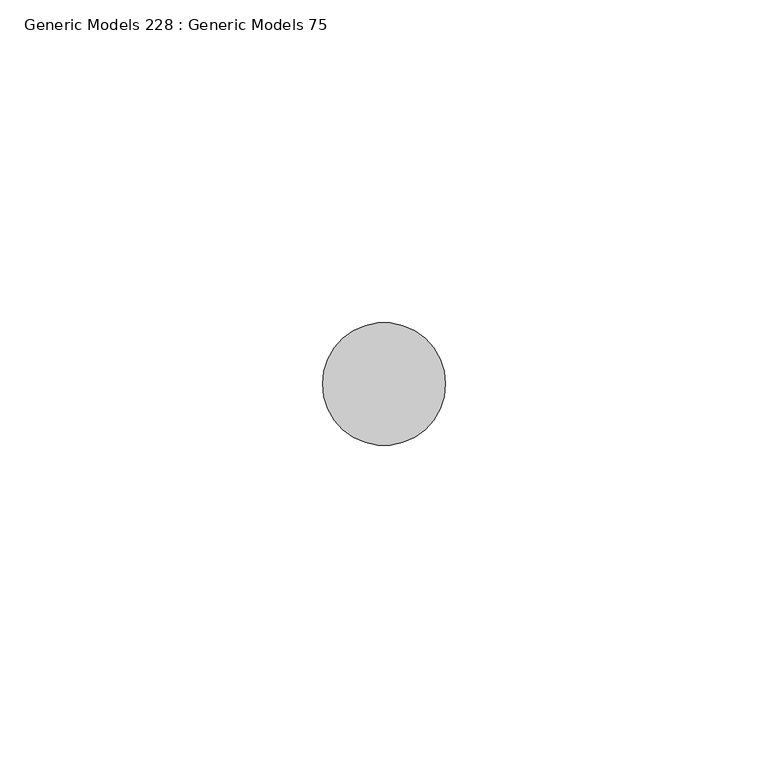
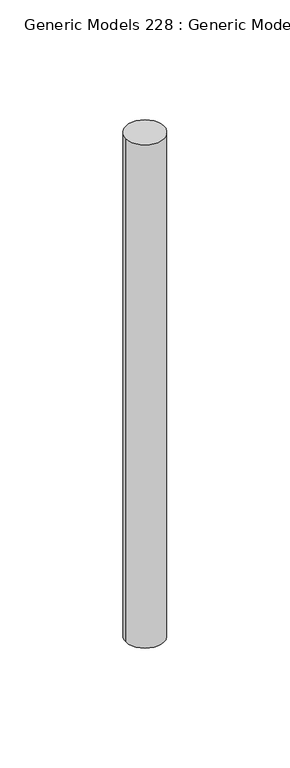
"""IFC4 building model written with IfcOpenShell, lengths in millimetres: proxy geometry, Generic Models 228 : Generic Models 75."""

from ifc_helpers import new_model, si_unit, point, frame, frame_2d, origin, place, context, project, spatial, circle_curve, trimmed, segment, composite_curve, outline, extrude, source, transform, mapped, element, save


def generic_models_228_generic_models_75_c9aeced4(model_context):
    return source(origin(), model_context, "Body", "SweptSolid", [
        extrude(outline(composite_curve([segment(trimmed(circle_curve(frame_2d((31988.1215778, 35167.5357185)), 9.525), [point((31978.5965778, 35167.5357185))], [point((31997.6465778, 35167.5357185))], False, "CARTESIAN"), True, "CONTINUOUS"), segment(trimmed(circle_curve(frame_2d((31988.1215778, 35167.5357185)), 9.525), [point((31997.6465778, 35167.5357185))], [point((31978.5965778, 35167.5357185))], False, "CARTESIAN"), True, "CONTINUOUS")], self_intersect=False)), frame((0.0, 0.0, 266172.95), z_axis=(0.0, 0.0, 1.0), x_axis=(1.0, 0.0, 0.0)), (0.0, 0.0, 1.0), 266.7),
    ])


if __name__ == "__main__":
    model = new_model("IFC4")
    model_context = context("Model", 3, world=origin())
    ifc_project = project(units=[si_unit("LENGTHUNIT", "METRE", prefix="MILLI")], contexts=[model_context])
    site = spatial("IfcSite", under=ifc_project)
    building = spatial("IfcBuilding", under=site)
    placement = place(None, origin())
    generic_models_228_generic_models_75_shape = generic_models_228_generic_models_75_c9aeced4(model_context)
    element("IfcBuildingElementProxy", 1, Name="Generic Models 228 : Generic Models 75", ObjectType="Generic Models 228 : Generic Models 75", at=placement, inside=building, context=model_context, shape_type="MappedRepresentation", body=[
        mapped(generic_models_228_generic_models_75_shape, transform((0.0, 0.0, 0.0), x_axis=(1.0, 0.0, 0.0), y_axis=(0.0, 1.0, 0.0), z_axis=(0.0, 0.0, 1.0))),
    ])
    save(model, "model.ifc")

# Revit data of these elements
# Element 1 (IfcBuildingElementProxy, "Generic Models 228 : Generic Models 75")
#   Materials on its faces: "5/8\" DIA. EPOXY ANCHOR BOLTS"
# Materials
#   "5/8\" DIA. EPOXY ANCHOR BOLTS": class "Metal", colour RGB 199 199 199, transparency 0, Description = "Carbon steel", Cost = 0
